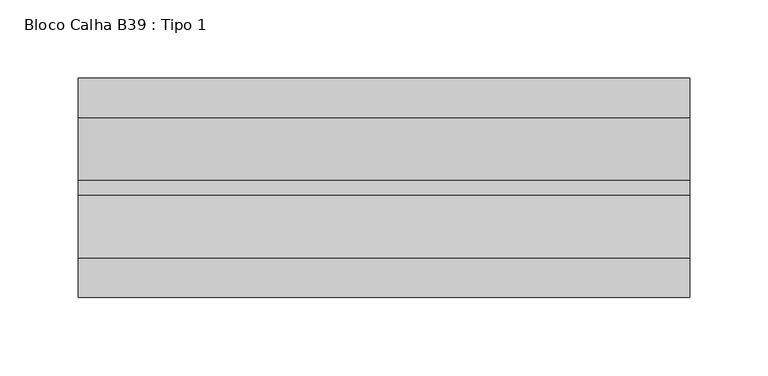
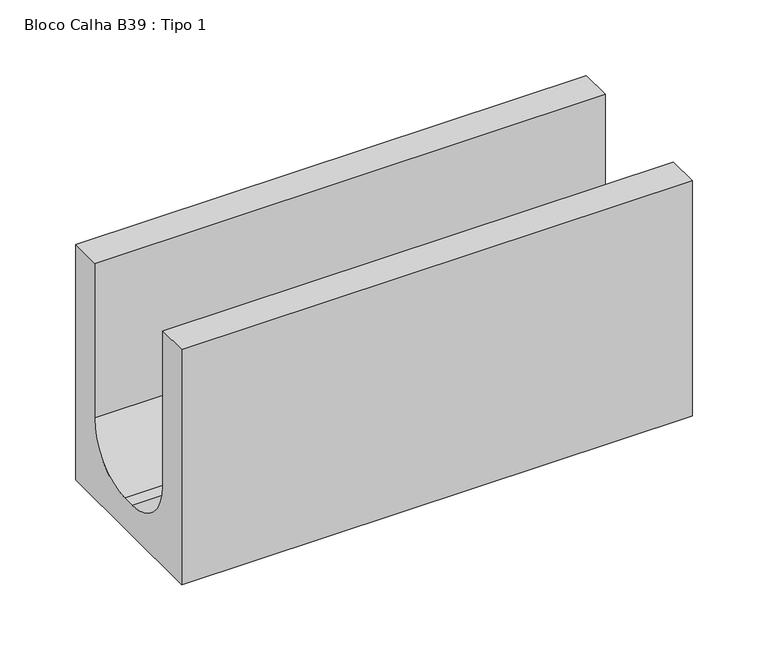
"""IFC4 building model written with IfcOpenShell, lengths in millimetres: proxy geometry, Bloco Calha B39 : Tipo 1."""

from ifc_helpers import new_model, si_unit, point, frame, frame_2d, origin, place, context, project, spatial, polyline, circle_curve, trimmed, segment, composite_curve, outline, extrude, source, transform, mapped, element, save


def bloco_calha_b39_tipo_1_a5fcad13(model_context):
    return source(origin(), model_context, "Body", "SweptSolid", [
        extrude(outline(composite_curve([segment(polyline([(140.0, 0.0), (0.0, 0.0), (0.0, 190.0), (25.0, 190.0), (25.0, 65.0)]), True, "CONTINUOUS"), segment(trimmed(circle_curve(frame_2d((65.0, 65.0)), 40.0), [point((25.0, 65.0))], [point((65.0, 25.0))], True, "CARTESIAN"), True, "CONTINUOUS"), segment(polyline([(65.0, 25.0), (75.0, 25.0)]), True, "CONTINUOUS"), segment(trimmed(circle_curve(frame_2d((75.0, 65.0)), 40.0), [point((75.0, 25.0))], [point((115.0, 65.0))], True, "CARTESIAN"), True, "CONTINUOUS"), segment(polyline([(115.0, 65.0), (115.0, 190.0), (140.0, 190.0), (140.0, 0.0)]), True, "CONTINUOUS")], self_intersect=False)), frame((0.0, 0.0, 0.0), z_axis=(1.0, 0.0, 0.0), x_axis=(0.0, 1.0, 0.0)), (0.0, 0.0, 1.0), 390.0),
    ])


if __name__ == "__main__":
    model = new_model("IFC4")
    model_context = context("Model", 3, world=origin())
    ifc_project = project(units=[si_unit("LENGTHUNIT", "METRE", prefix="MILLI")], contexts=[model_context])
    site = spatial("IfcSite", under=ifc_project)
    building = spatial("IfcBuilding", under=site)
    placement = place(None, origin())
    bloco_calha_b39_tipo_1_shape = bloco_calha_b39_tipo_1_a5fcad13(model_context)
    element("IfcBuildingElementProxy", 1, Name="Bloco Calha B39 : Tipo 1", ObjectType="Bloco Calha B39 : Tipo 1", at=placement, inside=building, context=model_context, shape_type="MappedRepresentation", body=[
        mapped(bloco_calha_b39_tipo_1_shape, transform((0.0, 0.0, 0.0), x_axis=(1.0, 0.0, 0.0), y_axis=(0.0, 1.0, 0.0), z_axis=(0.0, 0.0, 1.0))),
    ])
    save(model, "model.ifc")

# Revit data of these elements
# Type "Bloco Calha B39 : Tipo 1"
#   SINAPI = ""
#   Assembly Code = ""
